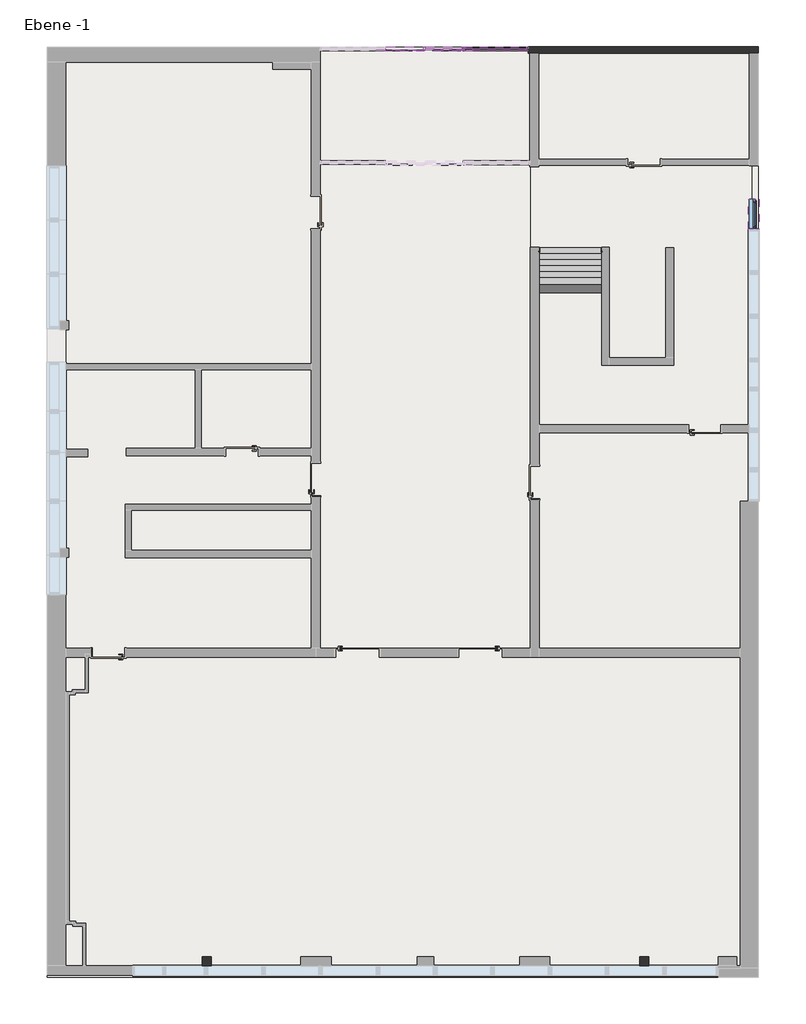
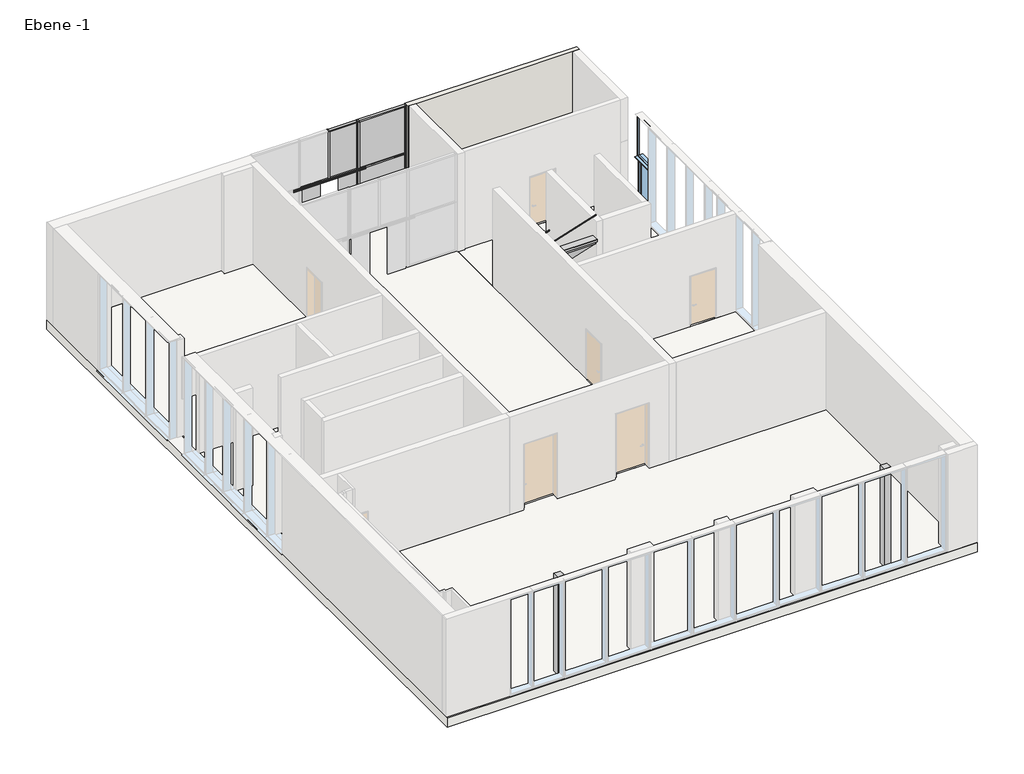
# One storey, part 3 of 3: 14 members, 8 slabs, 5 plates, 2 columns, 2 railings, 2 windows, 1 stair flight, 1 wall.
"""IFC4 building model written with IfcOpenShell, lengths in millimetres."""

import ifcopenshell
import ifcopenshell.guid

model = None  # the IFC model being written
_history = None  # IfcOwnerHistory: only IFC2X3 demands one
_inside = {}  # id of a spatial element -> (the spatial element, [elements in it])
_under = {}  # id of a project, library or spatial element -> (it, [spatial elements below it])
_declared = {}  # id of a project -> (the project, [libraries it declares])
_typed = {}  # id of a type object -> (the type object, [elements of that type])
_made_of = {}  # id of a material, layer set ... -> (it, [elements and type objects made of it])


def new_model(schema):
    """Start an empty IFC model of exactly this schema.

    Asked for "IFC4X3", IfcOpenShell would pick the latest addendum, in which some entities
    have other attributes; the version numbers below select the first issue.
    IFC2X3 requires an IfcOwnerHistory on every rooted entity: one is made here for all.
    """
    global model, _history
    if schema == "IFC4X3":
        model = ifcopenshell.file(schema_version=(4, 3, 0, 0))
    else:
        model = ifcopenshell.file(schema=schema)
    _inside.clear()
    _under.clear()
    _declared.clear()
    _typed.clear()
    _made_of.clear()
    _history = None
    if model.schema == "IFC2X3":
        org = make("IfcOrganization", Name="unknown")
        user = make(
            "IfcPersonAndOrganization",
            ThePerson=make("IfcPerson", FamilyName="unknown"),
            TheOrganization=org,
        )
        app = make(
            "IfcApplication",
            ApplicationDeveloper=org,
            Version="unknown",
            ApplicationFullName="unknown",
            ApplicationIdentifier="unknown",
        )
        _history = make(
            "IfcOwnerHistory",
            OwningUser=user,
            OwningApplication=app,
            ChangeAction="ADDED",
            CreationDate=0,
        )
    return model


def make(cls, **values):
    """One entity of the class cls with the attributes given. An attribute that is None is left unset."""
    return model.create_entity(
        cls, **{name: value for name, value in values.items() if value is not None}
    )


def rooted(cls, **values):
    """An entity with a GlobalId (a new one), such as an element, a storey or a relation."""
    return make(cls, GlobalId=ifcopenshell.guid.new(), OwnerHistory=_history, **values)


def si_unit(unit_type, name, prefix=None):
    """IfcSIUnit, for example si_unit("LENGTHUNIT", "METRE", prefix="MILLI")."""
    return make("IfcSIUnit", UnitType=unit_type, Prefix=prefix, Name=name)


def assignment(units):
    """IfcUnitAssignment: the units of a project."""
    return None if units is None else make("IfcUnitAssignment", Units=units)


def point(xyz):
    """IfcCartesianPoint."""
    return None if xyz is None else make("IfcCartesianPoint", Coordinates=xyz)


def direction(xyz):
    """IfcDirection."""
    return None if xyz is None else make("IfcDirection", DirectionRatios=xyz)


def frame(location, z_axis=None, x_axis=None):
    """IfcAxis2Placement3D, a coordinate frame: its origin and axes. An axis left out is left unset."""
    return make(
        "IfcAxis2Placement3D",
        Location=point(location),
        Axis=direction(z_axis),
        RefDirection=direction(x_axis),
    )


def origin():
    """The frame at (0, 0, 0) with its axes left unset."""
    return frame((0.0, 0.0, 0.0))


def origin_with_axes():
    """The frame at (0, 0, 0) with the z axis (0, 0, 1) and the x axis (1, 0, 0) written out."""
    return frame((0.0, 0.0, 0.0), z_axis=(0.0, 0.0, 1.0), x_axis=(1.0, 0.0, 0.0))


def place(relative_to, where):
    """IfcLocalPlacement: puts the frame where relative to a parent placement (None: the world)."""
    return make(
        "IfcLocalPlacement", PlacementRelTo=relative_to, RelativePlacement=where
    )


def context(
    kind, dimensions, precision=None, world=None, true_north=None, identifier=None
):
    """IfcGeometricRepresentationContext, for example the 3D "Model" context."""
    return make(
        "IfcGeometricRepresentationContext",
        ContextIdentifier=identifier,
        ContextType=kind,
        CoordinateSpaceDimension=dimensions,
        Precision=precision,
        WorldCoordinateSystem=world,
        TrueNorth=true_north,
    )


def project(units=None, contexts=None):
    """IfcProject with its units and contexts."""
    return rooted(
        "IfcProject",
        Name="project",
        RepresentationContexts=contexts,
        UnitsInContext=assignment(units),
    )


def spatial(cls, under=None, at=None, **own):
    """A site, building, storey or space (cls), placed at a placement, below another one or the project."""
    s = rooted(cls, ObjectPlacement=at, **own)
    if under is not None:
        _under.setdefault(under.id(), (under, []))[1].append(s)
    return s


def polyline(points):
    """IfcPolyline through the points."""
    return make("IfcPolyline", Points=[point(p) for p in points])


def ellipse_curve(where, semi_axis1, semi_axis2):
    """IfcEllipse in the frame where."""
    return make(
        "IfcEllipse", Position=where, SemiAxis1=semi_axis1, SemiAxis2=semi_axis2
    )


def outline(outer, holes=None, kind="AREA"):
    """IfcArbitraryClosedProfileDef: a profile drawn as a closed curve; with holes, ...WithVoids."""
    if holes is None:
        return make("IfcArbitraryClosedProfileDef", ProfileType=kind, OuterCurve=outer)
    return make(
        "IfcArbitraryProfileDefWithVoids",
        ProfileType=kind,
        OuterCurve=outer,
        InnerCurves=holes,
    )


def extrude(swept, where, along, depth):
    """IfcExtrudedAreaSolid: the profile swept, set in the frame where, extruded along a direction by depth."""
    return make(
        "IfcExtrudedAreaSolid",
        SweptArea=swept,
        Position=where,
        ExtrudedDirection=direction(along),
        Depth=depth,
    )


def faces_of(points, faces, orient=None, outer=None):
    """IfcFace entities. A face is a list of loops; a loop is a list of indices into points, from 0.

    orient and outer hold one flag for each loop. By default every Orientation is true, the
    first loop of a face is its IfcFaceOuterBound and the others are IfcFaceBound.
    """
    made = []
    for i, loops in enumerate(faces):
        bounds = []
        for j, loop in enumerate(loops):
            is_outer = j == 0 if outer is None else outer[i][j]
            bounds.append(
                make(
                    "IfcFaceOuterBound" if is_outer else "IfcFaceBound",
                    Bound=make("IfcPolyLoop", Polygon=[points[k] for k in loop]),
                    Orientation=True if orient is None else orient[i][j],
                )
            )
        made.append(make("IfcFace", Bounds=bounds))
    return made


def faceted_brep(points, faces, orient=None, outer=None, voids=None):
    """IfcFacetedBrep: a solid bounded by flat faces; with voids (closed shells), ...WithVoids."""
    shared = [point(p) for p in points]
    hull = make("IfcClosedShell", CfsFaces=faces_of(shared, faces, orient, outer))
    if voids is None:
        return make("IfcFacetedBrep", Outer=hull)
    return make(
        "IfcFacetedBrepWithVoids",
        Outer=hull,
        Voids=[
            make(cls, CfsFaces=faces_of(shared, fs, o, b)) for cls, fs, o, b in voids
        ],
    )


def shape(context_of_items, identifier, shape_type, items):
    """IfcShapeRepresentation: the items that make up one representation, for example the "Body"."""
    return make(
        "IfcShapeRepresentation",
        ContextOfItems=context_of_items,
        RepresentationIdentifier=identifier,
        RepresentationType=shape_type,
        Items=items,
    )


def source(mapping_origin, context_of_items, identifier, shape_type, items):
    """IfcRepresentationMap: a shape defined once, which mapped items show again and again."""
    return make(
        "IfcRepresentationMap",
        MappingOrigin=mapping_origin,
        MappedRepresentation=shape(context_of_items, identifier, shape_type, items),
    )


def transform(
    local_origin,
    x_axis=None,
    y_axis=None,
    z_axis=None,
    scale=None,
    scale2=None,
    scale3=None,
    uniform=True,
):
    """IfcCartesianTransformationOperator3D, or its non-uniform kind. x_axis, y_axis, z_axis: its Axis1, 2, 3."""
    if uniform:
        return make(
            "IfcCartesianTransformationOperator3D",
            Axis1=direction(x_axis),
            Axis2=direction(y_axis),
            LocalOrigin=point(local_origin),
            Scale=scale,
            Axis3=direction(z_axis),
        )
    return make(
        "IfcCartesianTransformationOperator3DnonUniform",
        Axis1=direction(x_axis),
        Axis2=direction(y_axis),
        LocalOrigin=point(local_origin),
        Scale=scale,
        Axis3=direction(z_axis),
        Scale2=scale2,
        Scale3=scale3,
    )


def mapped(mapping_source, mapping_target):
    """IfcMappedItem: shows the shape of a source again, moved by a transform."""
    return make(
        "IfcMappedItem", MappingSource=mapping_source, MappingTarget=mapping_target
    )


def made_of(thing, what):
    """Note that an element or type object is made of a material, layer set ...; save() writes the relation."""
    if what is not None:
        _made_of.setdefault(what.id(), (what, []))[1].append(thing)
    return thing


def element(
    cls,
    number,
    at=None,
    inside=None,
    cuts=None,
    type_object=None,
    material=None,
    context=None,
    identifier="Body",
    shape_type=None,
    held_by="IfcProductDefinitionShape",
    body=None,
    shapes=None,
    **own,
):
    """One element of the class cls, such as IfcWall. Its Tag is "e" and its number.

    at: its placement. inside: the storey or other place that contains it. cuts: it is an
    opening in that element (IfcRelVoidsElement). A single representation is given by context,
    identifier, shape_type and body (its items); several are given by shapes. held_by: the class
    of the entity that holds the representations. save() writes the other relations.
    """
    e = rooted(cls, Tag="e%d" % number, ObjectPlacement=at, **own)
    if body is not None:
        shapes = [shape(context, identifier, shape_type, body)]
    if shapes is not None:
        e.Representation = make(held_by, Representations=shapes)
    if inside is not None:
        _inside.setdefault(inside.id(), (inside, []))[1].append(e)
    if cuts is not None:
        rooted(
            "IfcRelVoidsElement", RelatingBuildingElement=cuts, RelatedOpeningElement=e
        )
    if type_object is not None:
        _typed.setdefault(type_object.id(), (type_object, []))[1].append(e)
    return made_of(e, material)


def aggregate(whole, parts):
    """IfcRelAggregates: a whole, such as a stair, and the parts it consists of."""
    return rooted("IfcRelAggregates", RelatingObject=whole, RelatedObjects=parts)


def save(model, path):
    """Write the relations noted so far, then the file.

    IfcRelAggregates (storeys below a building ...), IfcRelContainedInSpatialStructure (elements
    in a storey), IfcRelDefinesByType, IfcRelAssociatesMaterial and IfcRelDeclares: one each for
    every whole, place, type object, material and project.
    """
    for whole, parts in _under.values():
        aggregate(whole, parts)
    for where, things in _inside.values():
        rooted(
            "IfcRelContainedInSpatialStructure",
            RelatedElements=things,
            RelatingStructure=where,
        )
    for kind, things in _typed.values():
        rooted("IfcRelDefinesByType", RelatedObjects=things, RelatingType=kind)
    for what, things in _made_of.values():
        rooted("IfcRelAssociatesMaterial", RelatedObjects=things, RelatingMaterial=what)
    for by, libraries in _declared.values():
        rooted("IfcRelDeclares", RelatingContext=by, RelatedDefinitions=libraries)
    model.write(path)


def plane_surface(at):
    """IfcPlane: the flat surface through the origin of the frame at, square to its z axis."""
    return make("IfcPlane", Position=at)


def cylinder_surface(at, radius):
    """IfcCylindricalSurface: all points at the distance radius from the z axis of the frame at."""
    return make("IfcCylindricalSurface", Position=at, Radius=radius)


def advanced_brep(points, edges, surfaces, faces):
    """IfcAdvancedBrep: a solid bounded by faces that lie on surfaces and meet in shared edges.

    An edge is (start, end): straight between two places in points (the first is 0);
    or (start, end, curve); or (start, end, curve, False) where it runs against its curve.
    A face is (place in surfaces, loops), or (place, loops, False) where it looks against
    its surface's normal. A loop lists edges by number (the first is 1), with a minus sign
    where the edge is run from its end to its start. The first loop is the outer one.
    """
    corners = [point(p) for p in points]
    vertices = [make("IfcVertexPoint", VertexGeometry=c) for c in corners]
    made = []
    for start, end, *more in edges:
        made.append(
            make(
                "IfcEdgeCurve",
                EdgeStart=vertices[start],
                EdgeEnd=vertices[end],
                EdgeGeometry=more[0] if more else make("IfcPolyline", Points=[corners[start], corners[end]]),
                SameSense=more[1] if len(more) > 1 else True,
            )
        )
    hull = []
    for where, loops, *sense in faces:
        bounds = []
        for j, loop in enumerate(loops):
            ring = [make("IfcOrientedEdge", EdgeElement=made[abs(k) - 1], Orientation=k > 0) for k in loop]
            bounds.append(
                make(
                    "IfcFaceOuterBound" if j == 0 else "IfcFaceBound",
                    Bound=make("IfcEdgeLoop", EdgeList=ring),
                    Orientation=True,
                )
            )
        hull.append(make("IfcAdvancedFace", Bounds=bounds, FaceSurface=surfaces[where], SameSense=sense[0] if sense else True))
    return make("IfcAdvancedBrep", Outer=make("IfcClosedShell", CfsFaces=hull))


def stb_30_x_30_23a68b31(model_context):
    return source(origin(), model_context, "Body", "SweptSolid", [
        extrude(outline(polyline([(150.0, 150.0), (150.0, -150.0), (-150.0, -150.0), (-150.0, 150.0), (150.0, 150.0)])), frame((0.0, 0.0, -1584.8398838), z_axis=(0.0, 0.0, 1.0), x_axis=(1.0, 0.0, 0.0)), (0.0, 0.0, 1.0), 4584.8398838),
    ])


def pfosten_rechteckig_6_x_12_0a3b7900(model_context):
    return source(origin(), model_context, "Body", "SweptSolid", [
        extrude(outline(polyline([(0.0, 60.0), (0.0, -60.0), (-60.0, -60.0), (-60.0, 60.0), (0.0, 60.0)])), frame((0.0, 0.0, -2050.0000003), z_axis=(0.0, 0.0, 1.0), x_axis=(1.0, 0.0, 0.0)), (0.0, 0.0, 1.0), 2050.0000003),
    ])


def pfosten_rechteckig_6_x_12_07c25811(model_context):
    return source(origin(), model_context, "Body", "SweptSolid", [
        extrude(outline(polyline([(30.0, 60.0), (30.0, -60.0), (-30.0, -60.0), (-30.0, 60.0), (30.0, 60.0)])), frame((0.0, 0.0, -2050.0000003), z_axis=(0.0, 0.0, 1.0), x_axis=(1.0, 0.0, 0.0)), (0.0, 0.0, 1.0), 2050.0000003),
    ])


def pfosten_rechteckig_6_x_12_9195eeaf(model_context):
    return source(origin(), model_context, "Body", "SweptSolid", [
        extrude(outline(polyline([(0.0, 60.0), (0.0, -60.0), (-60.0, -60.0), (-60.0, 60.0), (0.0, 60.0)])), frame((0.0, 0.0, -1210.0000003), z_axis=(0.0, 0.0, 1.0), x_axis=(1.0, 0.0, 0.0)), (0.0, 0.0, 1.0), 1210.0000003),
    ])


def pfosten_rechteckig_6_x_12_f8cf5b5c(model_context):
    return source(origin(), model_context, "Body", "SweptSolid", [
        extrude(outline(polyline([(0.0, 60.0), (0.0, -60.0), (-60.0, -60.0), (-60.0, 60.0), (0.0, 60.0)])), frame((0.0, 0.0, -1240.0), z_axis=(0.0, 0.0, 1.0), x_axis=(1.0, 0.0, 0.0)), (0.0, 0.0, 1.0), 1240.0),
    ])


def pfosten_rechteckig_6_x_12_8a56a971(model_context):
    return source(origin(), model_context, "Body", "SweptSolid", [
        extrude(outline(polyline([(30.0, 60.0), (30.0, -60.0), (-30.0, -60.0), (-30.0, 60.0), (30.0, 60.0)])), frame((0.0, 0.0, -2320.0), z_axis=(0.0, 0.0, 1.0), x_axis=(1.0, 0.0, 0.0)), (0.0, 0.0, 1.0), 2320.0),
    ])


def pfosten_rechteckig_6_x_12_7e254c8a(model_context):
    return source(origin(), model_context, "Body", "SweptSolid", [
        extrude(outline(polyline([(0.0, 60.0), (0.0, -60.0), (-60.0, -60.0), (-60.0, 60.0), (0.0, 60.0)])), frame((0.0, 0.0, -2320.0), z_axis=(0.0, 0.0, 1.0), x_axis=(1.0, 0.0, 0.0)), (0.0, 0.0, 1.0), 2320.0),
    ])


def pfosten_rechteckig_6_x_12_09906e8b(model_context):
    return source(origin(), model_context, "Body", "SweptSolid", [
        extrude(outline(polyline([(30.0, 60.0), (30.0, -60.0), (-30.0, -60.0), (-30.0, 60.0), (30.0, 60.0)])), frame((0.0, 0.0, -2264.8398838), z_axis=(0.0, 0.0, 1.0), x_axis=(1.0, 0.0, 0.0)), (0.0, 0.0, 1.0), 2264.8398838),
    ])


def pfosten_rechteckig_6_x_12_b3245d14(model_context):
    return source(origin(), model_context, "Body", "SweptSolid", [
        extrude(outline(polyline([(0.0, 60.0), (0.0, -60.0), (-60.0, -60.0), (-60.0, 60.0), (0.0, 60.0)])), frame((0.0, 0.0, -2264.8398838), z_axis=(0.0, 0.0, 1.0), x_axis=(1.0, 0.0, 0.0)), (0.0, 0.0, 1.0), 2264.8398838),
    ])


def pfosten_rechteckig_6_x_12_6681f09f(model_context):
    return source(origin(), model_context, "Body", "SweptSolid", [
        extrude(outline(polyline([(30.0, 60.0), (30.0, -60.0), (-30.0, -60.0), (-30.0, 60.0), (30.0, 60.0)])), frame((0.0, 0.0, -2290.8558388), z_axis=(0.0, 0.0, 1.0), x_axis=(1.0, 0.0, 0.0)), (0.0, 0.0, 1.0), 2290.8558388),
    ])


def pfosten_rechteckig_6_x_12_74b065d3(model_context):
    return source(origin(), model_context, "Body", "SweptSolid", [
        extrude(outline(polyline([(0.0, 60.0), (0.0, -60.0), (-60.0, -60.0), (-60.0, 60.0), (0.0, 60.0)])), frame((0.0, 0.0, -2290.8558388), z_axis=(0.0, 0.0, 1.0), x_axis=(1.0, 0.0, 0.0)), (0.0, 0.0, 1.0), 2290.8558388),
    ])


def standard_dba1ab43(model_context):
    return source(origin(), model_context, "Body", "SweptSolid", [
        extrude(outline(polyline([(1200.0, -100.0), (1200.0, -130.0), (400.0, -130.0), (400.0, -100.0), (1200.0, -100.0)])), origin_with_axes(), (0.0, 0.0, 1.0), 2250.0),
        extrude(outline(polyline([(-400.0, -100.0), (-400.0, -130.0), (-1200.0, -130.0), (-1200.0, -100.0), (-400.0, -100.0)])), origin_with_axes(), (0.0, 0.0, 1.0), 2250.0),
        extrude(outline(polyline([(-140.0, 2295.0), (-140.0, 2250.0), (-145.0, 2250.0), (-145.0, 2300.0), (-85.0, 2300.0), (-85.0, 2250.0), (-90.0, 2250.0), (-90.0, 2295.0), (-140.0, 2295.0)])), frame((-1600.0, 0.0, 0.0), z_axis=(1.0, 0.0, 0.0), x_axis=(0.0, 1.0, 0.0)), (0.0, 0.0, 1.0), 3200.0),
    ])


def standard_af362adf(model_context):
    return source(origin(), model_context, "Body", "SweptSolid", [
        extrude(outline(polyline([(1200.0, -100.0), (1200.0, -130.0), (400.0, -130.0), (400.0, -100.0), (1200.0, -100.0)])), origin_with_axes(), (0.0, 0.0, 1.0), 43.984045),
        extrude(outline(polyline([(-400.0, -100.0), (-400.0, -130.0), (-1200.0, -130.0), (-1200.0, -100.0), (-400.0, -100.0)])), origin_with_axes(), (0.0, 0.0, 1.0), 43.984045),
        extrude(outline(polyline([(-140.0, 88.984045), (-140.0, 43.984045), (-145.0, 43.984045), (-145.0, 93.984045), (-85.0, 93.984045), (-85.0, 43.984045), (-90.0, 43.984045), (-90.0, 88.984045), (-140.0, 88.984045)])), frame((-1600.0, 0.0, 0.0), z_axis=(1.0, 0.0, 0.0), x_axis=(0.0, 1.0, 0.0)), (0.0, 0.0, 1.0), 3200.0),
    ])


def systemelement_verglasung_c088afcf(model_context):
    return source(origin(), model_context, "Body", "SweptSolid", [
        extrude(outline(polyline([(1025.0000002, -15.0), (-1025.0000002, -15.0), (-1025.0000002, 15.0), (1025.0000002, 15.0), (1025.0000002, -15.0)])), origin_with_axes(), (0.0, 0.0, 1.0), 2230.0),
    ])


def systemelement_verglasung_12e0d43f(model_context):
    return source(origin(), model_context, "Body", "SweptSolid", [
        extrude(outline(polyline([(1025.0000002, -15.0), (-1025.0000002, -15.0), (-1025.0000002, 15.0), (1025.0000002, 15.0), (1025.0000002, -15.0)])), origin_with_axes(), (0.0, 0.0, 1.0), 2174.8398838),
    ])


def systemelement_verglasung_f34c0457(model_context):
    return source(origin(), model_context, "Body", "SweptSolid", [
        extrude(outline(polyline([(605.0000002, -15.0), (-605.0000002, -15.0), (-605.0000002, 15.0), (605.0000002, 15.0), (605.0000002, -15.0)])), origin_with_axes(), (0.0, 0.0, 1.0), 2170.8558388),
    ])


def window_09175688(model_context):
    return source(origin(), model_context, "Body", "SweptSolid", [
        extrude(outline(polyline([(3000.0, 500.0), (3000.0, -500.0), (1000.0, -500.0), (1000.0, 500.0), (3000.0, 500.0)]), holes=[polyline([(2920.0, 440.0), (1080.0, 440.0), (1080.0, -440.0), (2920.0, -440.0), (2920.0, 440.0)])]), frame((0.0, 20.0, 0.0), z_axis=(0.0, 1.0, 0.0), x_axis=(0.0, 0.0, 1.0)), (0.0, 0.0, 1.0), 50.0),
        extrude(outline(polyline([(-500.0, -180.0), (-500.0, 20.0), (500.0, 20.0), (500.0, -180.0), (-500.0, -180.0)])), frame((0.0, 0.0, 1005.0), z_axis=(0.0, 0.0, 1.0), x_axis=(1.0, 0.0, 0.0)), (0.0, 0.0, 1.0), 15.0),
        extrude(outline(polyline([(80.0221543, 1020.0), (180.0, 1000.0), (180.0, 990.0), (178.0, 990.0), (178.0, 998.3604634), (79.8240723, 1018.0), (70.0, 1018.0), (70.0, 1020.0), (80.0221543, 1020.0)])), frame((-500.0, 0.0, 0.0), z_axis=(1.0, 0.0, 0.0), x_axis=(0.0, 1.0, 0.0)), (0.0, 0.0, 1.0), 1000.0),
    ])


def window_4f3e8dcf(model_context):
    return source(origin(), model_context, "Body", "SolidModel", [
        extrude(outline(polyline([(2600.0, 500.0), (2600.0, -500.0), (0.0, -500.0), (0.0, 500.0), (2600.0, 500.0)]), holes=[polyline([(2520.0, 420.0), (80.0, 420.0), (80.0, -420.0), (2520.0, -420.0), (2520.0, 420.0)])]), frame((0.0, -58.6893832, 0.0), z_axis=(0.0, 1.0, 0.0), x_axis=(0.0, 0.0, 1.0)), (0.0, 0.0, 1.0), 80.0),
        faceted_brep([(450.0, -58.6893832, 2550.0), (450.0, -88.6893832, 2550.0), (450.0, -88.6893832, 50.0), (450.0, -58.6893832, 50.0), (-450.0, -88.6893832, 2550.0), (-450.0, -88.6893832, 50.0), (390.0, -88.6893832, 110.0), (-390.0, -88.6893832, 110.0), (-390.0, -88.6893832, 2490.0), (390.0, -88.6893832, 2490.0), (-450.0, -58.6893832, 50.0), (-450.0, -58.6893832, 2550.0), (420.0, -58.6893832, 2520.0), (-420.0, -58.6893832, 2520.0), (-420.0, -58.6893832, 80.0), (420.0, -58.6893832, 80.0), (420.0, -28.6893832, 2520.0), (420.0, -28.6893832, 80.0), (-420.0, -28.6893832, 80.0), (-420.0, -28.6893832, 2520.0), (390.0, -28.6893832, 2490.0), (-390.0, -28.6893832, 2490.0), (-390.0, -28.6893832, 110.0), (390.0, -28.6893832, 110.0)], [[[0, 1, 2, 3]], [[1, 4, 5, 2], [6, 7, 8, 9]], [[3, 2, 5, 10]], [[3, 10, 11, 0], [12, 13, 14, 15]], [[16, 12, 15, 17]], [[17, 15, 14, 18]], [[17, 18, 19, 16], [20, 21, 22, 23]], [[9, 20, 23, 6]], [[6, 23, 22, 7]], [[10, 5, 4, 11]], [[18, 14, 13, 19]], [[7, 22, 21, 8]], [[11, 4, 1, 0]], [[19, 13, 12, 16]], [[8, 21, 20, 9]]]),
        extrude(outline(polyline([(31.3327711, 20.0), (180.0, 0.0), (180.0, -10.0), (178.0, -10.0), (178.0, -1.6395366), (31.1346891, 18.0), (21.3106168, 18.0), (21.3106168, 20.0), (31.3327711, 20.0)])), frame((-500.0, 0.0, 0.0), z_axis=(1.0, 0.0, 0.0), x_axis=(0.0, 1.0, 0.0)), (0.0, 0.0, 1.0), 1000.0),
        extrude(outline(polyline([(390.0, -73.6893832), (-390.0, -73.6893832), (-390.0, -43.6893832), (390.0, -43.6893832), (390.0, -73.6893832)])), frame((0.0, 0.0, 110.0), z_axis=(0.0, 0.0, 1.0), x_axis=(1.0, 0.0, 0.0)), (0.0, 0.0, 1.0), 2380.0),
    ])


model = new_model("IFC4")

# Units and contexts
model_context = context("Model", 3, world=origin())
ifc_project = project(units=[si_unit("LENGTHUNIT", "METRE", prefix="MILLI")], contexts=[model_context])

# Site, building, storey
site = spatial("IfcSite", under=ifc_project)
building = spatial("IfcBuilding", under=site)
storey = spatial("IfcBuildingStorey", under=building, Name="Ebene -1", Elevation=-1584.8398838)

# Columns
placement = place(None, origin())
stb_30_x_30_shape = stb_30_x_30_23a68b31(model_context)
element("IfcColumn", 1, ObjectType="STB Stütze - rechteckig : STB 30 x 30", at=placement, inside=storey, context=model_context, shape_type="MappedRepresentation", body=[
    mapped(stb_30_x_30_shape, transform((-6876.0626383, -16433.1054617, 0.0), x_axis=(1.0, 0.0, 0.0), y_axis=(0.0, 1.0, 0.0), z_axis=(0.0, 0.0, 1.0))),
])
element("IfcColumn", 2, ObjectType="STB Stütze - rechteckig : STB 30 x 30", at=placement, inside=storey, context=model_context, shape_type="MappedRepresentation", body=[
    mapped(stb_30_x_30_shape, transform((7633.9373617, -16438.1054617, 0.0), x_axis=(1.0, 0.0, 0.0), y_axis=(0.0, 1.0, 0.0), z_axis=(0.0, 0.0, 1.0))),
])

# Members
pfosten_rechteckig_6_x_12_shape = pfosten_rechteckig_6_x_12_0a3b7900(model_context)
element("IfcMember", 3, ObjectType="Pfosten rechteckig : 6 x 12", at=placement, inside=storey, context=model_context, shape_type="MappedRepresentation", body=[
    mapped(pfosten_rechteckig_6_x_12_shape, transform((1672.1636977, 13819.4184725, 3000.0), x_axis=(0.0, 0.0, 1.0), y_axis=(0.0, 1.0, 0.0), z_axis=(-1.0, 0.0, 0.0))),
])
element("IfcMember", 4, ObjectType="Pfosten rechteckig : 6 x 12", at=placement, inside=storey, context=model_context, shape_type="MappedRepresentation", body=[
    mapped(pfosten_rechteckig_6_x_12_shape, transform((3722.163698, 13819.4184725, -1584.8398838), x_axis=(0.0, 0.0, -1.0), y_axis=(0.0, 1.0, 0.0), z_axis=(1.0, 0.0, 0.0))),
])
pfosten_rechteckig_6_x_12_2_shape = pfosten_rechteckig_6_x_12_07c25811(model_context)
element("IfcMember", 5, ObjectType="Pfosten rechteckig : 6 x 12", at=placement, inside=storey, context=model_context, shape_type="MappedRepresentation", body=[
    mapped(pfosten_rechteckig_6_x_12_2_shape, transform((1672.1636977, 13819.4184725, 735.1601162), x_axis=(0.0, 0.0, 1.0), y_axis=(0.0, 1.0, 0.0), z_axis=(-1.0, 0.0, 0.0))),
])
pfosten_rechteckig_6_x_12_3_shape = pfosten_rechteckig_6_x_12_9195eeaf(model_context)
element("IfcMember", 6, ObjectType="Pfosten rechteckig : 6 x 12", at=placement, inside=storey, context=model_context, shape_type="MappedRepresentation", body=[
    mapped(pfosten_rechteckig_6_x_12_3_shape, transform((1574.3378966, 13819.4184725, 709.1441612), x_axis=(0.0, 0.0, -1.0), y_axis=(0.0, 1.0, 0.0), z_axis=(1.0, 0.0, 0.0))),
])
element("IfcMember", 7, ObjectType="Pfosten rechteckig : 6 x 12", at=placement, inside=storey, context=model_context, shape_type="MappedRepresentation", body=[
    mapped(pfosten_rechteckig_6_x_12_3_shape, transform((364.3378962, 13819.4184725, 3000.0), x_axis=(0.0, 0.0, 1.0), y_axis=(0.0, 1.0, 0.0), z_axis=(-1.0, 0.0, 0.0))),
])
pfosten_rechteckig_6_x_12_4_shape = pfosten_rechteckig_6_x_12_f8cf5b5c(model_context)
element("IfcMember", 8, ObjectType="Pfosten rechteckig : 6 x 12", at=placement, inside=storey, context=model_context, shape_type="MappedRepresentation", body=[
    mapped(pfosten_rechteckig_6_x_12_4_shape, transform((304.3378962, 13819.4184725, 709.1441612), x_axis=(0.0, 0.0, -1.0), y_axis=(0.0, 1.0, 0.0), z_axis=(1.0, 0.0, 0.0))),
])
pfosten_rechteckig_6_x_12_5_shape = pfosten_rechteckig_6_x_12_8a56a971(model_context)
element("IfcMember", 9, ObjectType="Pfosten rechteckig : 6 x 12", at=placement, inside=storey, context=model_context, shape_type="MappedRepresentation", body=[
    mapped(pfosten_rechteckig_6_x_12_5_shape, transform((1642.1636977, 13819.4184725, -1584.8398838), x_axis=(-1.0, 0.0, 0.0), y_axis=(0.0, 1.0, 0.0), z_axis=(0.0, 0.0, -1.0))),
])
pfosten_rechteckig_6_x_12_6_shape = pfosten_rechteckig_6_x_12_7e254c8a(model_context)
element("IfcMember", 10, ObjectType="Pfosten rechteckig : 6 x 12", at=placement, inside=storey, context=model_context, shape_type="MappedRepresentation", body=[
    mapped(pfosten_rechteckig_6_x_12_6_shape, transform((1634.3378966, 13819.4184725, -1584.8398838), x_axis=(-1.0, 0.0, 0.0), y_axis=(0.0, 1.0, 0.0), z_axis=(0.0, 0.0, -1.0))),
])
element("IfcMember", 11, ObjectType="Pfosten rechteckig : 6 x 12", at=placement, inside=storey, context=model_context, shape_type="MappedRepresentation", body=[
    mapped(pfosten_rechteckig_6_x_12_6_shape, transform((3782.163698, 13819.4184725, 735.1601162), x_axis=(1.0, 0.0, 0.0), y_axis=(0.0, 1.0, 0.0), z_axis=(0.0, 0.0, 1.0))),
])
pfosten_rechteckig_6_x_12_7_shape = pfosten_rechteckig_6_x_12_09906e8b(model_context)
element("IfcMember", 12, ObjectType="Pfosten rechteckig : 6 x 12", at=placement, inside=storey, context=model_context, shape_type="MappedRepresentation", body=[
    mapped(pfosten_rechteckig_6_x_12_7_shape, transform((1642.1636977, 13819.4184725, 735.1601162), x_axis=(-1.0, 0.0, 0.0), y_axis=(0.0, 1.0, 0.0), z_axis=(0.0, 0.0, -1.0))),
])
pfosten_rechteckig_6_x_12_8_shape = pfosten_rechteckig_6_x_12_b3245d14(model_context)
element("IfcMember", 13, ObjectType="Pfosten rechteckig : 6 x 12", at=placement, inside=storey, context=model_context, shape_type="MappedRepresentation", body=[
    mapped(pfosten_rechteckig_6_x_12_8_shape, transform((3782.163698, 13819.4184725, 3000.0), x_axis=(1.0, 0.0, 0.0), y_axis=(0.0, 1.0, 0.0), z_axis=(0.0, 0.0, 1.0))),
])
element("IfcMember", 14, ObjectType="Pfosten rechteckig : 6 x 12", at=placement, inside=storey, context=model_context, shape_type="MappedRepresentation", body=[
    mapped(pfosten_rechteckig_6_x_12_8_shape, transform((1634.3378966, 13819.4184725, 735.1601162), x_axis=(-1.0, 0.0, 0.0), y_axis=(0.0, 1.0, 0.0), z_axis=(0.0, 0.0, -1.0))),
])
pfosten_rechteckig_6_x_12_9_shape = pfosten_rechteckig_6_x_12_6681f09f(model_context)
element("IfcMember", 15, ObjectType="Pfosten rechteckig : 6 x 12", at=placement, inside=storey, context=model_context, shape_type="MappedRepresentation", body=[
    mapped(pfosten_rechteckig_6_x_12_9_shape, transform((334.3378962, 13819.4184725, 709.1441612), x_axis=(-1.0, 0.0, 0.0), y_axis=(0.0, 1.0, 0.0), z_axis=(0.0, 0.0, -1.0))),
])
pfosten_rechteckig_6_x_12_10_shape = pfosten_rechteckig_6_x_12_74b065d3(model_context)
element("IfcMember", 16, ObjectType="Pfosten rechteckig : 6 x 12", at=placement, inside=storey, context=model_context, shape_type="MappedRepresentation", body=[
    mapped(pfosten_rechteckig_6_x_12_10_shape, transform((1634.3378966, 13819.4184725, 3000.0), x_axis=(1.0, 0.0, 0.0), y_axis=(0.0, 1.0, 0.0), z_axis=(0.0, 0.0, 1.0))),
])

# Plates
standard_shape = standard_dba1ab43(model_context)
element("IfcPlate", 17, ObjectType="Türelement 2-flg - Schiebeflügel : Standard", at=placement, inside=storey, context=model_context, shape_type="MappedRepresentation", body=[
    mapped(standard_shape, transform((344.9611791, 13879.4184725, -1584.8398838), x_axis=(1.0, 0.0, 0.0), y_axis=(0.0, 1.0, 0.0), z_axis=(0.0, 0.0, 1.0))),
])
standard_2_shape = standard_af362adf(model_context)
element("IfcPlate", 18, ObjectType="Türelement 2-flg - Schiebeflügel : Standard", at=placement, inside=storey, context=model_context, shape_type="MappedRepresentation", body=[
    mapped(standard_2_shape, transform((344.9611791, 13879.4184725, 665.1601162), x_axis=(1.0, 0.0, 0.0), y_axis=(0.0, 1.0, 0.0), z_axis=(0.0, 0.0, 1.0))),
])
systemelement_verglasung_shape = systemelement_verglasung_c088afcf(model_context)
element("IfcPlate", 19, ObjectType="Systemelement : Verglasung", at=placement, inside=storey, context=model_context, shape_type="MappedRepresentation", body=[
    mapped(systemelement_verglasung_shape, transform((2697.1636979, 13819.4184725, -1524.8398838), x_axis=(-1.0, 0.0, 0.0), y_axis=(0.0, -1.0, 0.0), z_axis=(0.0, 0.0, 1.0))),
])
systemelement_verglasung_2_shape = systemelement_verglasung_12e0d43f(model_context)
element("IfcPlate", 20, ObjectType="Systemelement : Verglasung", at=placement, inside=storey, context=model_context, shape_type="MappedRepresentation", body=[
    mapped(systemelement_verglasung_2_shape, transform((2697.1636979, 13819.4184725, 765.1601162), x_axis=(-1.0, 0.0, 0.0), y_axis=(0.0, -1.0, 0.0), z_axis=(0.0, 0.0, 1.0))),
])
systemelement_verglasung_3_shape = systemelement_verglasung_f34c0457(model_context)
element("IfcPlate", 21, ObjectType="Systemelement : Verglasung", at=placement, inside=storey, context=model_context, shape_type="MappedRepresentation", body=[
    mapped(systemelement_verglasung_3_shape, transform((969.3378964, 13819.4184725, 769.1441612), x_axis=(-1.0, 0.0, 0.0), y_axis=(0.0, -1.0, 0.0), z_axis=(0.0, 0.0, 1.0))),
])

# Railings
element("IfcRailing", 22, ObjectType="Holzhandlauf", at=placement, inside=storey, context=model_context, shape_type="AdvancedBrep", body=[
    advanced_brep(
    [(4129.7988542, 7221.3974899, -514.8854908), (4169.7988542, 7221.3974899, -514.8854908), (4129.7988542, 3421.3974899, 3249.1092333), (4169.7988542, 3421.3974899, 3249.1092333)],
    [
        (0, 1, ellipse_curve(frame((4149.7988542, 7221.3974899, -514.8854908), z_axis=(0.0, 1.0, 0.0), x_axis=(0.0, 0.0, -1.0)), 28.1505924, 20.0)),
        (1, 0, ellipse_curve(frame((4149.7988542, 7221.3974899, -514.8854908), z_axis=(0.0, 1.0, 0.0), x_axis=(0.0, 0.0, -1.0)), 28.1505924, 20.0)),
        (2, 3, ellipse_curve(frame((4149.7988542, 3421.3974899, 3249.1092333), z_axis=(0.0, -1.0, 0.0), x_axis=(0.0, 0.0, -1.0)), 28.1505924, 20.0)),
        (3, 2, ellipse_curve(frame((4149.7988542, 3421.3974899, 3249.1092333), z_axis=(0.0, -1.0, 0.0), x_axis=(0.0, 0.0, -1.0)), 28.1505924, 20.0)),
        (0, 2),
        (3, 1),
    ],
    [
        plane_surface(frame((4149.7988542, 7221.3974899, -486.7348983), z_axis=(0.0, 1.0, 0.0), x_axis=(0.0, 0.0, -1.0))),
        plane_surface(frame((4149.7988542, 3421.3974899, 3277.2598257), z_axis=(0.0, -1.0, 0.0), x_axis=(0.0, 0.0, -1.0))),
        cylinder_surface(frame((4149.7988542, 7207.3228315, -500.9441908), z_axis=(0.0, 0.7104646222980373, -0.703732918416431), x_axis=(1.0, 0.0, 0.0)), 20.0),
    ],
    [
        (0, [[1, 2]]),
        (1, [[3, 4]]),
        (2, [[-1, 5, -4, 6]]),
        (2, [[-2, -6, -3, -5]]),
    ],
),
])
element("IfcRailing", 23, ObjectType="Holzhandlauf", at=placement, inside=storey, context=model_context, shape_type="AdvancedBrep", body=[
    advanced_brep(
    [(6203.5701306, 7221.3974899, -514.8854908), (6243.5701306, 7221.3974899, -514.8854908), (6203.5701306, 3421.3974899, 3249.1092333), (6243.5701306, 3421.3974899, 3249.1092333)],
    [
        (0, 1, ellipse_curve(frame((6223.5701306, 7221.3974899, -514.8854908), z_axis=(0.0, 1.0, 0.0), x_axis=(0.0, 0.0, -1.0)), 28.1505924, 20.0)),
        (1, 0, ellipse_curve(frame((6223.5701306, 7221.3974899, -514.8854908), z_axis=(0.0, 1.0, 0.0), x_axis=(0.0, 0.0, -1.0)), 28.1505924, 20.0)),
        (2, 3, ellipse_curve(frame((6223.5701306, 3421.3974899, 3249.1092333), z_axis=(0.0, -1.0, 0.0), x_axis=(0.0, 0.0, -1.0)), 28.1505924, 20.0)),
        (3, 2, ellipse_curve(frame((6223.5701306, 3421.3974899, 3249.1092333), z_axis=(0.0, -1.0, 0.0), x_axis=(0.0, 0.0, -1.0)), 28.1505924, 20.0)),
        (0, 2),
        (3, 1),
    ],
    [
        plane_surface(frame((6223.5701306, 7221.3974899, -486.7348983), z_axis=(0.0, 1.0, 0.0), x_axis=(0.0, 0.0, -1.0))),
        plane_surface(frame((6223.5701306, 3421.3974899, 3277.2598257), z_axis=(0.0, -1.0, 0.0), x_axis=(0.0, 0.0, -1.0))),
        cylinder_surface(frame((6223.5701306, 7207.3228315, -500.9441908), z_axis=(0.0, 0.7104646222980384, -0.7037329184164299), x_axis=(1.0, 0.0, 0.0)), 20.0),
    ],
    [
        (0, [[1, 2]]),
        (1, [[3, 4]]),
        (2, [[-1, 5, -4, 6]]),
        (2, [[-2, -6, -3, -5]]),
    ],
),
])

# Slabs
element("IfcSlab", 24, ObjectType="Fließen", at=placement, inside=storey, context=model_context, shape_type="SweptSolid", body=[
    extrude(outline(polyline([(4149.3988542, -3.0186326), (4149.3988542, 1096.5309721), (11109.7002114, 1096.5309721), (11109.7002114, -1190.3664069), (10812.1787516, -1190.3664069), (10812.1787516, -6055.798296), (4149.3988542, -6055.798296), (4149.3988542, -1125.8186326), (3849.3988542, -1125.8186326), (3849.3988542, -3.0186326), (4149.3988542, -3.0186326)])), frame((0.0, 0.0, -1604.8398838), z_axis=(0.0, 0.0, 1.0), x_axis=(1.0, 0.0, 0.0)), (0.0, 0.0, 1.0), 20.0),
])
element("IfcSlab", 25, ObjectType="PVC", at=placement, inside=storey, context=model_context, shape_type="SweptSolid", body=[
    extrude(outline(polyline([(-3102.8646224, 96.7587617), (-3102.8646224, 13764.201704), (3769.3333907, 13764.201704), (3769.3333907, 13684.201704), (3849.3333907, 13684.201704), (3849.3333907, -6055.798296), (2949.3333907, -6055.798296), (1449.3333907, -6055.798296), (-1131.4646224, -6055.798296), (-2631.4646224, -6055.798296), (-3102.8646224, -6055.798296), (-3102.8646224, -1026.0412383), (-3402.8646224, -1026.0412383), (-3402.8646224, 96.7587617), (-3102.8646224, 96.7587617)])), frame((0.0, 0.0, -1604.8398838), z_axis=(0.0, 0.0, 1.0), x_axis=(1.0, 0.0, 0.0)), (0.0, 0.0, 1.0), 20.0),
])
element("IfcSlab", 26, ObjectType="PVC", at=placement, inside=storey, context=model_context, shape_type="SweptSolid", body=[
    extrude(outline(polyline([(4149.3988542, 7231.701704), (3849.3333907, 7231.701704), (3849.3333907, 9907.1335931), (4132.0873617, 9907.1335931), (4132.0873617, 9954.6335931), (11192.1787516, 9954.6335931), (11192.1787516, 7851.3974899), (11109.7988542, 7851.3974899), (11109.7988542, 1351.3974899), (10189.7988542, 1351.3974899), (10189.7988542, 1091.3974899), (9069.7988542, 1091.3974899), (9069.7988542, 1351.3974899), (4129.7988542, 1351.3974899), (4129.7988542, 7111.3974899), (6223.9701306, 7111.3974899), (6223.9701306, 3331.3974899), (8603.9701306, 3331.3974899), (8603.9701306, 7228.0387191), (8353.9701306, 7228.0387191), (8353.9701306, 3581.3974899), (6473.9701306, 3581.3974899), (6473.9701306, 7231.3974899), (6223.9701306, 7231.3974899), (6223.9701306, 7221.3974899), (4149.3988542, 7221.3974899), (4149.3988542, 7231.701704)])), frame((0.0, 0.0, -1604.8398838), z_axis=(0.0, 0.0, 1.0), x_axis=(1.0, 0.0, 0.0)), (0.0, 0.0, 1.0), 20.0),
])
element("IfcSlab", 27, ObjectType="PVC", at=placement, inside=storey, context=model_context, shape_type="SweptSolid", body=[
    extrude(outline(polyline([(11112.1787516, 13679.6335931), (11112.1787516, 10157.1335931), (8188.5330566, 10157.1335931), (8188.5330566, 9957.1335931), (7065.7330566, 9957.1335931), (7065.7330566, 10157.1335931), (4132.0873617, 10157.1335931), (4132.0873617, 13679.6335931), (11112.1787516, 13679.6335931)])), frame((0.0, 0.0, -1604.8398838), z_axis=(0.0, 0.0, 1.0), x_axis=(1.0, 0.0, 0.0)), (0.0, 0.0, 1.0), 20.0),
])
element("IfcSlab", 28, ObjectType="PVC", at=placement, inside=storey, context=model_context, shape_type="SweptSolid", body=[
    extrude(outline(polyline([(-3402.8646224, 3372.9613782), (-11555.5781798, 3372.9613782), (-11555.5781798, 3367.8804464), (-11775.5781798, 3367.8804464), (-11775.5781798, 3422.8804464), (-11786.8887966, 3422.8804464), (-11946.8887966, 3422.8804464), (-11946.8887966, 4549.0661003), (-11751.3453606, 4549.0661003), (-11751.3453606, 4509.0661003), (-11451.3453606, 4509.0661003), (-11451.3453606, 4807.8804464), (-11775.5781798, 4807.8804464), (-11775.5781798, 9942.8804464), (-11552.1836955, 9942.8804464), (-11552.1836955, 13359.7901533), (-4677.1836955, 13359.7901533), (-4677.1836955, 13134.7901533), (-3402.8646224, 13134.7901533), (-3402.8646224, 8951.9741313), (-3102.8646224, 8951.9741313), (-3102.8646224, 7829.1741313), (-3402.8646224, 7829.1741313), (-3402.8646224, 3372.9613782)])), frame((0.0, 0.0, -1604.8398838), z_axis=(0.0, 0.0, 1.0), x_axis=(1.0, 0.0, 0.0)), (0.0, 0.0, 1.0), 20.0),
])
element("IfcSlab", 29, ObjectType="PVC", at=placement, inside=storey, context=model_context, shape_type="SweptSolid", body=[
    extrude(outline(polyline([(-7248.9898594, 3172.9613782), (-7248.9898594, 576.7587617), (-9542.7330305, 576.7587617), (-9542.7330305, 326.7587617), (-6265.6646224, 326.7587617), (-6265.6646224, 576.7587617), (-7048.9898594, 576.7587617), (-7048.9898594, 3172.9613782), (-3402.8646224, 3172.9613782), (-3402.8646224, 576.7587617), (-5142.8646224, 576.7587617), (-5142.8646224, 326.7587617), (-3402.8646224, 326.7587617), (-3402.8646224, -1283.2412383), (-9577.9707378, -1283.2412383), (-9577.9707378, -3057.6984082), (-3402.8646224, -3057.6984082), (-3402.8646224, -6055.798296), (-9572.7781798, -6055.798296), (-9572.7781798, -6355.798296), (-10695.5781798, -6355.798296), (-10695.5781798, -6055.798296), (-11555.5781798, -6055.798296), (-11555.5781798, -4280.798296), (-11741.4463914, -4280.798296), (-11771.4463914, -4280.798296), (-11771.4463914, -3030.798296), (-11442.1859447, -3030.798296), (-11442.1859447, -2736.5083915), (-11771.4463914, -2736.5083915), (-11771.4463914, 296.1078694), (-10820.3655355, 296.1078694), (-10820.3655355, 546.1078694), (-11771.4463914, 546.1078694), (-11771.4463914, 3172.9613782), (-7248.9898594, 3172.9613782)])), frame((0.0, 0.0, -1604.8398838), z_axis=(0.0, 0.0, 1.0), x_axis=(1.0, 0.0, 0.0)), (0.0, 0.0, 1.0), 20.0),
])
element("IfcSlab", 30, ObjectType="Parkett", at=placement, inside=storey, context=model_context, shape_type="SweptSolid", body=[
    extrude(outline(polyline([(-11555.5781798, -16592.4902923), (-11555.5781798, -6355.798296), (-2631.4646224, -6355.798296), (-2631.4646224, -6055.798296), (-1127.8646224, -6055.798296), (-1127.8646224, -6355.798296), (1449.3333907, -6355.798296), (1449.3333907, -6055.798296), (2949.3988542, -6055.798296), (2949.3988542, -6355.798296), (10812.1787516, -6355.798296), (10812.1787516, -16592.4902923), (-11555.5781798, -16592.4902923)])), frame((0.0, 0.0, -1604.8398838), z_axis=(0.0, 0.0, 1.0), x_axis=(1.0, 0.0, 0.0)), (0.0, 0.0, 1.0), 20.0),
])
element("IfcSlab", 31, ObjectType="STB 30", at=placement, inside=storey, context=model_context, shape_type="SweptSolid", body=[
    extrude(outline(polyline([(11412.1787516, 13869.4184725), (11412.1787516, -16973.0988284), (-12157.8212484, -16973.0988284), (-12157.8212484, 13869.4184725), (11412.1787516, 13869.4184725)])), frame((0.0, 0.0, -2024.8398838), z_axis=(0.0, 0.0, 1.0), x_axis=(1.0, 0.0, 0.0)), (0.0, 0.0, 1.0), 420.0),
])

# Stair flight
element("IfcStairFlight", 32, ObjectType="Holzauftritt 30 mm, Trittüberstand 30 mm", at=placement, inside=storey, context=model_context, shape_type="SolidModel", body=[
    faceted_brep([(6223.9701306, 6991.3974899, -1416.7348983), (6223.9701306, 7191.3974899, -1416.7348983), (4149.3988542, 7191.3974899, -1416.7348983), (4149.3988542, 6991.3974899, -1416.7348983), (6223.9701306, 6991.3974899, -1584.8398838), (6223.9701306, 7191.3974899, -1584.8398838), (4149.3988542, 7191.3974899, -1584.8398838), (4149.3988542, 6991.3974899, -1584.8398838), (6223.9701306, 6791.3974899, -1218.6299129), (6223.9701306, 6991.3974899, -1218.6299129), (4149.3988542, 6991.3974899, -1218.6299129), (4149.3988542, 6791.3974899, -1218.6299129), (6223.9701306, 6791.3974899, -1429.7593559), (6223.9701306, 6947.9614729, -1584.8398838), (4149.3988542, 6947.9614729, -1584.8398838), (4149.3988542, 6791.3974899, -1429.7593559), (6223.9701306, 6591.3974899, -1020.5249274), (6223.9701306, 6791.3974899, -1020.5249274), (4149.3988542, 6791.3974899, -1020.5249274), (4149.3988542, 6591.3974899, -1020.5249274), (6223.9701306, 6591.3974899, -1231.6543704), (4149.3988542, 6591.3974899, -1231.6543704), (6223.9701306, 6391.3974899, -822.4199419), (6223.9701306, 6591.3974899, -822.4199419), (4149.3988542, 6591.3974899, -822.4199419), (4149.3988542, 6391.3974899, -822.4199419), (6223.9701306, 6391.3974899, -1033.5493849), (4149.3988542, 6391.3974899, -1033.5493849), (6223.9701306, 6191.3974899, -624.3149564), (6223.9701306, 6391.3974899, -624.3149564), (4149.3988542, 6391.3974899, -624.3149564), (4149.3988542, 6191.3974899, -624.3149564), (6223.9701306, 6191.3974899, -835.4443995), (4149.3988542, 6191.3974899, -835.4443995), (6223.9701306, 5991.3974899, -426.209971), (6223.9701306, 6191.3974899, -426.209971), (4149.3988542, 6191.3974899, -426.209971), (4149.3988542, 5991.3974899, -426.209971), (6223.9701306, 5991.3974899, -637.339414), (4149.3988542, 5991.3974899, -637.339414), (6223.9701306, 5791.3974899, -228.1049855), (6223.9701306, 5991.3974899, -228.1049855), (4149.3988542, 5991.3974899, -228.1049855), (4149.3988542, 5791.3974899, -228.1049855), (6223.9701306, 5791.3974899, -439.2344285), (4149.3988542, 5791.3974899, -439.2344285), (6223.9701306, 5591.3974899, -241.129443), (6223.9701306, 5391.3974899, -43.0244576), (6223.9701306, 5191.3974899, 155.0805279), (6223.9701306, 4991.3974899, 353.1855134), (6223.9701306, 4791.3974899, 551.2904989), (6223.9701306, 4591.3974899, 749.3954844), (6223.9701306, 4391.3974899, 947.5004698), (6223.9701306, 4191.3974899, 1145.6054553), (6223.9701306, 3991.3974899, 1343.7104408), (6223.9701306, 3791.3974899, 1541.8154263), (6223.9701306, 3591.3974899, 1739.9204118), (6223.9701306, 3421.3974899, 1908.3096494), (4149.3988542, 3421.3974899, 1908.3096494), (4149.3988542, 3591.3974899, 1739.9204118), (4149.3988542, 3791.3974899, 1541.8154263), (4149.3988542, 3991.3974899, 1343.7104408), (4149.3988542, 4191.3974899, 1145.6054553), (4149.3988542, 4391.3974899, 947.5004698), (4149.3988542, 4591.3974899, 749.3954844), (4149.3988542, 4791.3974899, 551.2904989), (4149.3988542, 4991.3974899, 353.1855134), (4149.3988542, 5191.3974899, 155.0805279), (4149.3988542, 5391.3974899, -43.0244576), (4149.3988542, 5591.3974899, -241.129443), (4149.3988542, 3321.3974899, 2049.1548403), (4149.3988542, 3421.3974899, 2049.1548403), (6223.9701306, 3421.3974899, 2049.1548403), (6223.9701306, 3321.3974899, 2049.1548403), (6223.9701306, 3321.3974899, 2149.1548403), (4149.3988542, 3321.3974899, 2149.1548403), (6223.9701306, 5591.3974899, -30.0), (6223.9701306, 5791.3974899, -30.0), (4149.3988542, 5791.3974899, -30.0), (4149.3988542, 5591.3974899, -30.0), (6223.9701306, 5391.3974899, 168.1049855), (6223.9701306, 5591.3974899, 168.1049855), (4149.3988542, 5591.3974899, 168.1049855), (4149.3988542, 5391.3974899, 168.1049855), (6223.9701306, 5191.3974899, 366.209971), (6223.9701306, 5391.3974899, 366.209971), (4149.3988542, 5391.3974899, 366.209971), (4149.3988542, 5191.3974899, 366.209971), (6223.9701306, 4991.3974899, 564.3149564), (6223.9701306, 5191.3974899, 564.3149564), (4149.3988542, 5191.3974899, 564.3149564), (4149.3988542, 4991.3974899, 564.3149564), (6223.9701306, 4791.3974899, 762.4199419), (6223.9701306, 4991.3974899, 762.4199419), (4149.3988542, 4991.3974899, 762.4199419), (4149.3988542, 4791.3974899, 762.4199419), (6223.9701306, 4591.3974899, 960.5249274), (6223.9701306, 4791.3974899, 960.5249274), (4149.3988542, 4791.3974899, 960.5249274), (4149.3988542, 4591.3974899, 960.5249274), (6223.9701306, 4391.3974899, 1158.6299129), (6223.9701306, 4591.3974899, 1158.6299129), (4149.3988542, 4591.3974899, 1158.6299129), (4149.3988542, 4391.3974899, 1158.6299129), (6223.9701306, 4191.3974899, 1356.7348983), (6223.9701306, 4391.3974899, 1356.7348983), (4149.3988542, 4391.3974899, 1356.7348983), (4149.3988542, 4191.3974899, 1356.7348983), (6223.9701306, 3991.3974899, 1554.8398838), (6223.9701306, 4191.3974899, 1554.8398838), (4149.3988542, 4191.3974899, 1554.8398838), (4149.3988542, 3991.3974899, 1554.8398838), (6223.9701306, 3791.3974899, 1752.9448693), (6223.9701306, 3991.3974899, 1752.9448693), (4149.3988542, 3991.3974899, 1752.9448693), (4149.3988542, 3791.3974899, 1752.9448693), (6223.9701306, 3591.3974899, 1951.0498548), (6223.9701306, 3791.3974899, 1951.0498548), (4149.3988542, 3791.3974899, 1951.0498548), (4149.3988542, 3591.3974899, 1951.0498548), (6223.9701306, 3591.3974899, 2149.1548403), (4149.3988542, 3591.3974899, 2149.1548403)], [[[0, 1, 2, 3]], [[1, 0, 4, 5]], [[2, 1, 5, 6]], [[3, 2, 6, 7]], [[8, 9, 10, 11]], [[4, 0, 9, 8, 12, 13]], [[0, 3, 10, 9]], [[3, 7, 14, 15, 11, 10]], [[16, 17, 18, 19]], [[17, 16, 20, 12, 8]], [[8, 11, 18, 17]], [[19, 18, 11, 15, 21]], [[22, 23, 24, 25]], [[23, 22, 26, 20, 16]], [[16, 19, 24, 23]], [[25, 24, 19, 21, 27]], [[28, 29, 30, 31]], [[29, 28, 32, 26, 22]], [[22, 25, 30, 29]], [[31, 30, 25, 27, 33]], [[34, 35, 36, 37]], [[35, 34, 38, 32, 28]], [[28, 31, 36, 35]], [[37, 36, 31, 33, 39]], [[40, 41, 42, 43]], [[41, 40, 44, 38, 34]], [[34, 37, 42, 41]], [[43, 42, 37, 39, 45]], [[5, 4, 13, 14, 7, 6]], [[14, 13, 12, 20, 26, 32, 38, 44, 46, 47, 48, 49, 50, 51, 52, 53, 54, 55, 56, 57, 58, 59, 60, 61, 62, 63, 64, 65, 66, 67, 68, 69, 45, 39, 33, 27, 21, 15]], [[70, 71, 72, 73]], [[70, 73, 74, 75]], [[76, 77, 78, 79]], [[77, 76, 46, 44, 40]], [[40, 43, 78, 77]], [[79, 78, 43, 45, 69]], [[80, 81, 82, 83]], [[81, 80, 47, 46, 76]], [[76, 79, 82, 81]], [[83, 82, 79, 69, 68]], [[84, 85, 86, 87]], [[85, 84, 48, 47, 80]], [[80, 83, 86, 85]], [[87, 86, 83, 68, 67]], [[88, 89, 90, 91]], [[89, 88, 49, 48, 84]], [[84, 87, 90, 89]], [[91, 90, 87, 67, 66]], [[92, 93, 94, 95]], [[93, 92, 50, 49, 88]], [[88, 91, 94, 93]], [[95, 94, 91, 66, 65]], [[96, 97, 98, 99]], [[97, 96, 51, 50, 92]], [[92, 95, 98, 97]], [[99, 98, 95, 65, 64]], [[100, 101, 102, 103]], [[101, 100, 52, 51, 96]], [[96, 99, 102, 101]], [[103, 102, 99, 64, 63]], [[104, 105, 106, 107]], [[105, 104, 53, 52, 100]], [[100, 103, 106, 105]], [[107, 106, 103, 63, 62]], [[108, 109, 110, 111]], [[109, 108, 54, 53, 104]], [[104, 107, 110, 109]], [[111, 110, 107, 62, 61]], [[112, 113, 114, 115]], [[113, 112, 55, 54, 108]], [[108, 111, 114, 113]], [[115, 114, 111, 61, 60]], [[116, 117, 118, 119]], [[117, 116, 56, 55, 112]], [[112, 115, 118, 117]], [[119, 118, 115, 60, 59]], [[120, 121, 75, 74]], [[120, 74, 73, 72, 57, 56, 116]], [[116, 119, 121, 120]], [[75, 121, 119, 59, 58, 71, 70]], [[58, 57, 72, 71]]]),
    extrude(outline(polyline([(6223.9701306, 6991.3974899), (4149.3988542, 6991.3974899), (4149.3988542, 7221.3974899), (6223.9701306, 7221.3974899), (6223.9701306, 6991.3974899)])), frame((0.0, 0.0, -1416.7348983), z_axis=(0.0, 0.0, 1.0), x_axis=(1.0, 0.0, 0.0)), (0.0, 0.0, 1.0), 30.0),
    extrude(outline(polyline([(6223.9701306, 6791.3974899), (4149.3988542, 6791.3974899), (4149.3988542, 7021.3974899), (6223.9701306, 7021.3974899), (6223.9701306, 6791.3974899)])), frame((0.0, 0.0, -1218.6299129), z_axis=(0.0, 0.0, 1.0), x_axis=(1.0, 0.0, 0.0)), (0.0, 0.0, 1.0), 30.0),
    extrude(outline(polyline([(6223.9701306, 6591.3974899), (4149.3988542, 6591.3974899), (4149.3988542, 6821.3974899), (6223.9701306, 6821.3974899), (6223.9701306, 6591.3974899)])), frame((0.0, 0.0, -1020.5249274), z_axis=(0.0, 0.0, 1.0), x_axis=(1.0, 0.0, 0.0)), (0.0, 0.0, 1.0), 30.0),
    extrude(outline(polyline([(6223.9701306, 6391.3974899), (4149.3988542, 6391.3974899), (4149.3988542, 6621.3974899), (6223.9701306, 6621.3974899), (6223.9701306, 6391.3974899)])), frame((0.0, 0.0, -822.4199419), z_axis=(0.0, 0.0, 1.0), x_axis=(1.0, 0.0, 0.0)), (0.0, 0.0, 1.0), 30.0),
    extrude(outline(polyline([(6223.9701306, 6191.3974899), (4149.3988542, 6191.3974899), (4149.3988542, 6421.3974899), (6223.9701306, 6421.3974899), (6223.9701306, 6191.3974899)])), frame((0.0, 0.0, -624.3149564), z_axis=(0.0, 0.0, 1.0), x_axis=(1.0, 0.0, 0.0)), (0.0, 0.0, 1.0), 30.0),
    extrude(outline(polyline([(6223.9701306, 5991.3974899), (4149.3988542, 5991.3974899), (4149.3988542, 6221.3974899), (6223.9701306, 6221.3974899), (6223.9701306, 5991.3974899)])), frame((0.0, 0.0, -426.209971), z_axis=(0.0, 0.0, 1.0), x_axis=(1.0, 0.0, 0.0)), (0.0, 0.0, 1.0), 30.0),
    extrude(outline(polyline([(6223.9701306, 5791.3974899), (4149.3988542, 5791.3974899), (4149.3988542, 6021.3974899), (6223.9701306, 6021.3974899), (6223.9701306, 5791.3974899)])), frame((0.0, 0.0, -228.1049855), z_axis=(0.0, 0.0, 1.0), x_axis=(1.0, 0.0, 0.0)), (0.0, 0.0, 1.0), 30.0),
    extrude(outline(polyline([(6223.9701306, 5591.3974899), (4149.3988542, 5591.3974899), (4149.3988542, 5821.3974899), (6223.9701306, 5821.3974899), (6223.9701306, 5591.3974899)])), frame((0.0, 0.0, -30.0), z_axis=(0.0, 0.0, 1.0), x_axis=(1.0, 0.0, 0.0)), (0.0, 0.0, 1.0), 30.0),
    extrude(outline(polyline([(6223.9701306, 5391.3974899), (4149.3988542, 5391.3974899), (4149.3988542, 5621.3974899), (6223.9701306, 5621.3974899), (6223.9701306, 5391.3974899)])), frame((0.0, 0.0, 168.1049855), z_axis=(0.0, 0.0, 1.0), x_axis=(1.0, 0.0, 0.0)), (0.0, 0.0, 1.0), 30.0),
    extrude(outline(polyline([(6223.9701306, 5191.3974899), (4149.3988542, 5191.3974899), (4149.3988542, 5421.3974899), (6223.9701306, 5421.3974899), (6223.9701306, 5191.3974899)])), frame((0.0, 0.0, 366.209971), z_axis=(0.0, 0.0, 1.0), x_axis=(1.0, 0.0, 0.0)), (0.0, 0.0, 1.0), 30.0),
    extrude(outline(polyline([(6223.9701306, 4991.3974899), (4149.3988542, 4991.3974899), (4149.3988542, 5221.3974899), (6223.9701306, 5221.3974899), (6223.9701306, 4991.3974899)])), frame((0.0, 0.0, 564.3149564), z_axis=(0.0, 0.0, 1.0), x_axis=(1.0, 0.0, 0.0)), (0.0, 0.0, 1.0), 30.0),
    extrude(outline(polyline([(6223.9701306, 4791.3974899), (4149.3988542, 4791.3974899), (4149.3988542, 5021.3974899), (6223.9701306, 5021.3974899), (6223.9701306, 4791.3974899)])), frame((0.0, 0.0, 762.4199419), z_axis=(0.0, 0.0, 1.0), x_axis=(1.0, 0.0, 0.0)), (0.0, 0.0, 1.0), 30.0),
    extrude(outline(polyline([(6223.9701306, 4591.3974899), (4149.3988542, 4591.3974899), (4149.3988542, 4821.3974899), (6223.9701306, 4821.3974899), (6223.9701306, 4591.3974899)])), frame((0.0, 0.0, 960.5249274), z_axis=(0.0, 0.0, 1.0), x_axis=(1.0, 0.0, 0.0)), (0.0, 0.0, 1.0), 30.0),
    extrude(outline(polyline([(6223.9701306, 4391.3974899), (4149.3988542, 4391.3974899), (4149.3988542, 4621.3974899), (6223.9701306, 4621.3974899), (6223.9701306, 4391.3974899)])), frame((0.0, 0.0, 1158.6299129), z_axis=(0.0, 0.0, 1.0), x_axis=(1.0, 0.0, 0.0)), (0.0, 0.0, 1.0), 30.0),
    extrude(outline(polyline([(6223.9701306, 4191.3974899), (4149.3988542, 4191.3974899), (4149.3988542, 4421.3974899), (6223.9701306, 4421.3974899), (6223.9701306, 4191.3974899)])), frame((0.0, 0.0, 1356.7348983), z_axis=(0.0, 0.0, 1.0), x_axis=(1.0, 0.0, 0.0)), (0.0, 0.0, 1.0), 30.0),
    extrude(outline(polyline([(6223.9701306, 3991.3974899), (4149.3988542, 3991.3974899), (4149.3988542, 4221.3974899), (6223.9701306, 4221.3974899), (6223.9701306, 3991.3974899)])), frame((0.0, 0.0, 1554.8398838), z_axis=(0.0, 0.0, 1.0), x_axis=(1.0, 0.0, 0.0)), (0.0, 0.0, 1.0), 30.0),
    extrude(outline(polyline([(6223.9701306, 3791.3974899), (4149.3988542, 3791.3974899), (4149.3988542, 4021.3974899), (6223.9701306, 4021.3974899), (6223.9701306, 3791.3974899)])), frame((0.0, 0.0, 1752.9448693), z_axis=(0.0, 0.0, 1.0), x_axis=(1.0, 0.0, 0.0)), (0.0, 0.0, 1.0), 30.0),
    extrude(outline(polyline([(6223.9701306, 3591.3974899), (4149.3988542, 3591.3974899), (4149.3988542, 3821.3974899), (6223.9701306, 3821.3974899), (6223.9701306, 3591.3974899)])), frame((0.0, 0.0, 1951.0498548), z_axis=(0.0, 0.0, 1.0), x_axis=(1.0, 0.0, 0.0)), (0.0, 0.0, 1.0), 30.0),
    extrude(outline(polyline([(6223.9701306, 3321.3974899), (4149.3988542, 3321.3974899), (4149.3988542, 3621.3974899), (6223.9701306, 3621.3974899), (6223.9701306, 3321.3974899)])), frame((0.0, 0.0, 2149.1548403), z_axis=(0.0, 0.0, 1.0), x_axis=(1.0, 0.0, 0.0)), (0.0, 0.0, 1.0), 30.0),
])

# Wall
element("IfcWall", 33, ObjectType="STB 21.0 - Sichtbeton 1", at=placement, inside=storey, context=model_context, shape_type="Brep", body=[
    faceted_brep([(3782.163698, 13679.6335931, -1584.8398838), (3832.0873617, 13679.6335931, -1584.8398838), (4132.0873617, 13679.6335931, -1584.8398838), (11412.1787516, 13679.6335931, -1584.8398838), (11412.1787516, 13679.6335931, 3000.0), (4132.0873617, 13679.6335931, 3000.0), (3832.0873617, 13679.6335931, 3000.0), (3782.163698, 13679.6335931, 3000.0), (3782.163698, 13894.6335931, -1584.8398838), (3782.163698, 13894.6335931, 3000.0), (11412.1787516, 13894.6335931, 3000.0), (11412.1787516, 13894.6335931, -1584.8398838)], [[[0, 1, 2, 3, 4, 5, 6, 7]], [[8, 9, 10, 11]], [[3, 2, 1, 0, 8, 11]], [[0, 7, 9, 8]], [[4, 3, 11, 10]], [[7, 6, 5, 4, 10, 9]]]),
])

# Windows
window_shape = window_09175688(model_context)
element("IfcWindow", 34, ObjectType="Fenster - Festverglasung : Feste Verglasung 1.0 x2 2", at=placement, inside=storey, context=model_context, shape_type="MappedRepresentation", body=[
    mapped(window_shape, transform((11262.1787516, 8334.6335931, -4.0632904), x_axis=(0.0, 1.0, 0.0), y_axis=(-1.0, 0.0, 0.0), z_axis=(0.0, 0.0, 1.0))),
])
window_2_shape = window_4f3e8dcf(model_context)
element("IfcWindow", 35, ObjectType="Fenstertür 1-flg : 1.80 x  1", at=placement, inside=storey, context=model_context, shape_type="MappedRepresentation", body=[
    mapped(window_2_shape, transform((11262.1787516, 8329.6335931, -1589.0632904), x_axis=(0.0, 1.0, 0.0), y_axis=(-1.0, 0.0, 0.0), z_axis=(0.0, 0.0, 1.0))),
])

save(model, "model.ifc")

# Revit data of these elements
# Project information
#   Projektausgabedatum = "Projekt Datum"
